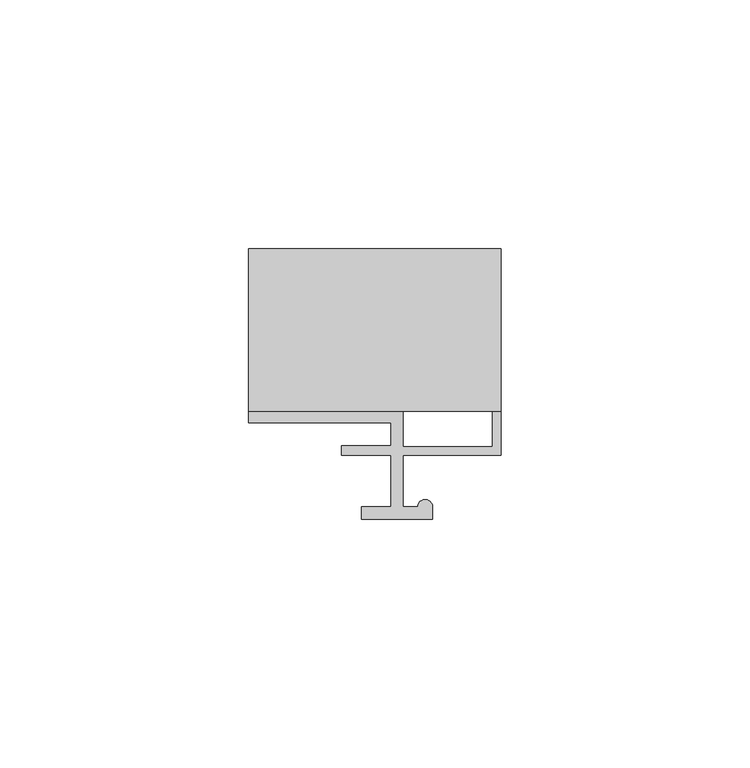
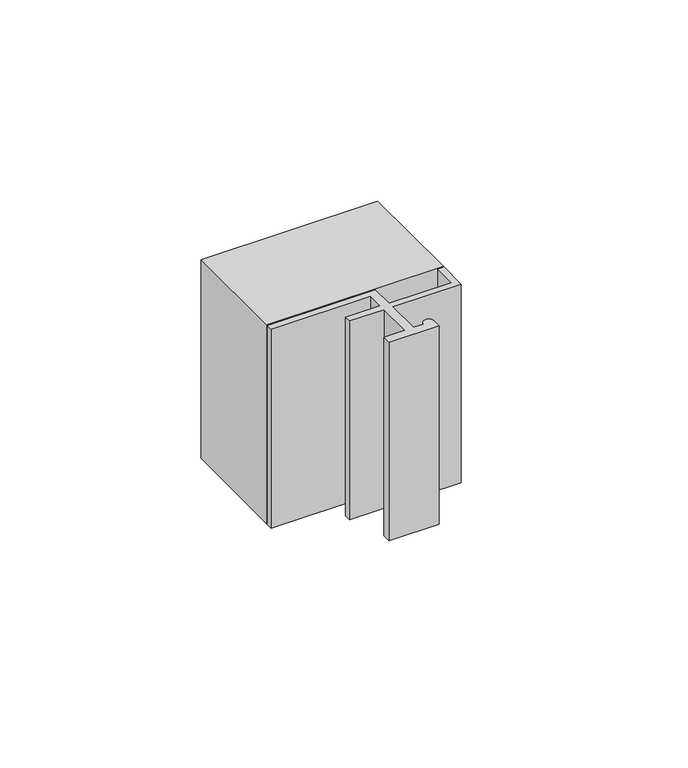
"""IFC4 building model written with IfcOpenShell, lengths in millimetres: proxy geometry, Generic Models 9:Generic Models 5:348123:Generic Models 5:348123 : Generic Models 9:Generic Models 5:348123:2 : Generic Models 9:Generic Models 5:348123:Generic Models 5:348123 : Generic Models 9:Generic Models 5:348123:301771."""

import ifcopenshell
import ifcopenshell.guid

model = None  # the IFC model being written
_history = None  # IfcOwnerHistory: only IFC2X3 demands one
_inside = {}  # id of a spatial element -> (the spatial element, [elements in it])
_under = {}  # id of a project, library or spatial element -> (it, [spatial elements below it])
_declared = {}  # id of a project -> (the project, [libraries it declares])
_typed = {}  # id of a type object -> (the type object, [elements of that type])
_made_of = {}  # id of a material, layer set ... -> (it, [elements and type objects made of it])


def new_model(schema):
    """Start an empty IFC model of exactly this schema.

    Asked for "IFC4X3", IfcOpenShell would pick the latest addendum, in which some entities
    have other attributes; the version numbers below select the first issue.
    IFC2X3 requires an IfcOwnerHistory on every rooted entity: one is made here for all.
    """
    global model, _history
    if schema == "IFC4X3":
        model = ifcopenshell.file(schema_version=(4, 3, 0, 0))
    else:
        model = ifcopenshell.file(schema=schema)
    _inside.clear()
    _under.clear()
    _declared.clear()
    _typed.clear()
    _made_of.clear()
    _history = None
    if model.schema == "IFC2X3":
        org = make("IfcOrganization", Name="unknown")
        user = make(
            "IfcPersonAndOrganization",
            ThePerson=make("IfcPerson", FamilyName="unknown"),
            TheOrganization=org,
        )
        app = make(
            "IfcApplication",
            ApplicationDeveloper=org,
            Version="unknown",
            ApplicationFullName="unknown",
            ApplicationIdentifier="unknown",
        )
        _history = make(
            "IfcOwnerHistory",
            OwningUser=user,
            OwningApplication=app,
            ChangeAction="ADDED",
            CreationDate=0,
        )
    return model


def make(cls, **values):
    """One entity of the class cls with the attributes given. An attribute that is None is left unset."""
    return model.create_entity(
        cls, **{name: value for name, value in values.items() if value is not None}
    )


def rooted(cls, **values):
    """An entity with a GlobalId (a new one), such as an element, a storey or a relation."""
    return make(cls, GlobalId=ifcopenshell.guid.new(), OwnerHistory=_history, **values)


def si_unit(unit_type, name, prefix=None):
    """IfcSIUnit, for example si_unit("LENGTHUNIT", "METRE", prefix="MILLI")."""
    return make("IfcSIUnit", UnitType=unit_type, Prefix=prefix, Name=name)


def assignment(units):
    """IfcUnitAssignment: the units of a project."""
    return None if units is None else make("IfcUnitAssignment", Units=units)


def point(xyz):
    """IfcCartesianPoint."""
    return None if xyz is None else make("IfcCartesianPoint", Coordinates=xyz)


def direction(xyz):
    """IfcDirection."""
    return None if xyz is None else make("IfcDirection", DirectionRatios=xyz)


def frame(location, z_axis=None, x_axis=None):
    """IfcAxis2Placement3D, a coordinate frame: its origin and axes. An axis left out is left unset."""
    return make(
        "IfcAxis2Placement3D",
        Location=point(location),
        Axis=direction(z_axis),
        RefDirection=direction(x_axis),
    )


def frame_2d(location, x_axis=None):
    """IfcAxis2Placement2D, a coordinate frame in the plane: its origin and x axis."""
    return make(
        "IfcAxis2Placement2D", Location=point(location), RefDirection=direction(x_axis)
    )


def origin():
    """The frame at (0, 0, 0) with its axes left unset."""
    return frame((0.0, 0.0, 0.0))


def place(relative_to, where):
    """IfcLocalPlacement: puts the frame where relative to a parent placement (None: the world)."""
    return make(
        "IfcLocalPlacement", PlacementRelTo=relative_to, RelativePlacement=where
    )


def context(
    kind, dimensions, precision=None, world=None, true_north=None, identifier=None
):
    """IfcGeometricRepresentationContext, for example the 3D "Model" context."""
    return make(
        "IfcGeometricRepresentationContext",
        ContextIdentifier=identifier,
        ContextType=kind,
        CoordinateSpaceDimension=dimensions,
        Precision=precision,
        WorldCoordinateSystem=world,
        TrueNorth=true_north,
    )


def project(units=None, contexts=None):
    """IfcProject with its units and contexts."""
    return rooted(
        "IfcProject",
        Name="project",
        RepresentationContexts=contexts,
        UnitsInContext=assignment(units),
    )


def spatial(cls, under=None, at=None, **own):
    """A site, building, storey or space (cls), placed at a placement, below another one or the project."""
    s = rooted(cls, ObjectPlacement=at, **own)
    if under is not None:
        _under.setdefault(under.id(), (under, []))[1].append(s)
    return s


def polyline(points):
    """IfcPolyline through the points."""
    return make("IfcPolyline", Points=[point(p) for p in points])


def circle_curve(where, radius):
    """IfcCircle in the frame where."""
    return make("IfcCircle", Position=where, Radius=radius)


def trimmed(basis, trim1, trim2, sense, master):
    """IfcTrimmedCurve: the piece of a basis curve between two trims."""
    return make(
        "IfcTrimmedCurve",
        BasisCurve=basis,
        Trim1=trim1,
        Trim2=trim2,
        SenseAgreement=sense,
        MasterRepresentation=master,
    )


def segment(curve, same_sense, transition):
    """IfcCompositeCurveSegment."""
    return make(
        "IfcCompositeCurveSegment",
        Transition=transition,
        SameSense=same_sense,
        ParentCurve=curve,
    )


def composite_curve(segments, self_intersect=None):
    """IfcCompositeCurve: segments joined end to end."""
    return make("IfcCompositeCurve", Segments=segments, SelfIntersect=self_intersect)


def outline(outer, holes=None, kind="AREA"):
    """IfcArbitraryClosedProfileDef: a profile drawn as a closed curve; with holes, ...WithVoids."""
    if holes is None:
        return make("IfcArbitraryClosedProfileDef", ProfileType=kind, OuterCurve=outer)
    return make(
        "IfcArbitraryProfileDefWithVoids",
        ProfileType=kind,
        OuterCurve=outer,
        InnerCurves=holes,
    )


def extrude(swept, where, along, depth):
    """IfcExtrudedAreaSolid: the profile swept, set in the frame where, extruded along a direction by depth."""
    return make(
        "IfcExtrudedAreaSolid",
        SweptArea=swept,
        Position=where,
        ExtrudedDirection=direction(along),
        Depth=depth,
    )


def shape(context_of_items, identifier, shape_type, items):
    """IfcShapeRepresentation: the items that make up one representation, for example the "Body"."""
    return make(
        "IfcShapeRepresentation",
        ContextOfItems=context_of_items,
        RepresentationIdentifier=identifier,
        RepresentationType=shape_type,
        Items=items,
    )


def source(mapping_origin, context_of_items, identifier, shape_type, items):
    """IfcRepresentationMap: a shape defined once, which mapped items show again and again."""
    return make(
        "IfcRepresentationMap",
        MappingOrigin=mapping_origin,
        MappedRepresentation=shape(context_of_items, identifier, shape_type, items),
    )


def transform(
    local_origin,
    x_axis=None,
    y_axis=None,
    z_axis=None,
    scale=None,
    scale2=None,
    scale3=None,
    uniform=True,
):
    """IfcCartesianTransformationOperator3D, or its non-uniform kind. x_axis, y_axis, z_axis: its Axis1, 2, 3."""
    if uniform:
        return make(
            "IfcCartesianTransformationOperator3D",
            Axis1=direction(x_axis),
            Axis2=direction(y_axis),
            LocalOrigin=point(local_origin),
            Scale=scale,
            Axis3=direction(z_axis),
        )
    return make(
        "IfcCartesianTransformationOperator3DnonUniform",
        Axis1=direction(x_axis),
        Axis2=direction(y_axis),
        LocalOrigin=point(local_origin),
        Scale=scale,
        Axis3=direction(z_axis),
        Scale2=scale2,
        Scale3=scale3,
    )


def mapped(mapping_source, mapping_target):
    """IfcMappedItem: shows the shape of a source again, moved by a transform."""
    return make(
        "IfcMappedItem", MappingSource=mapping_source, MappingTarget=mapping_target
    )


def made_of(thing, what):
    """Note that an element or type object is made of a material, layer set ...; save() writes the relation."""
    if what is not None:
        _made_of.setdefault(what.id(), (what, []))[1].append(thing)
    return thing


def element(
    cls,
    number,
    at=None,
    inside=None,
    cuts=None,
    type_object=None,
    material=None,
    context=None,
    identifier="Body",
    shape_type=None,
    held_by="IfcProductDefinitionShape",
    body=None,
    shapes=None,
    **own,
):
    """One element of the class cls, such as IfcWall. Its Tag is "e" and its number.

    at: its placement. inside: the storey or other place that contains it. cuts: it is an
    opening in that element (IfcRelVoidsElement). A single representation is given by context,
    identifier, shape_type and body (its items); several are given by shapes. held_by: the class
    of the entity that holds the representations. save() writes the other relations.
    """
    e = rooted(cls, Tag="e%d" % number, ObjectPlacement=at, **own)
    if body is not None:
        shapes = [shape(context, identifier, shape_type, body)]
    if shapes is not None:
        e.Representation = make(held_by, Representations=shapes)
    if inside is not None:
        _inside.setdefault(inside.id(), (inside, []))[1].append(e)
    if cuts is not None:
        rooted(
            "IfcRelVoidsElement", RelatingBuildingElement=cuts, RelatedOpeningElement=e
        )
    if type_object is not None:
        _typed.setdefault(type_object.id(), (type_object, []))[1].append(e)
    return made_of(e, material)


def aggregate(whole, parts):
    """IfcRelAggregates: a whole, such as a stair, and the parts it consists of."""
    return rooted("IfcRelAggregates", RelatingObject=whole, RelatedObjects=parts)


def save(model, path):
    """Write the relations noted so far, then the file.

    IfcRelAggregates (storeys below a building ...), IfcRelContainedInSpatialStructure (elements
    in a storey), IfcRelDefinesByType, IfcRelAssociatesMaterial and IfcRelDeclares: one each for
    every whole, place, type object, material and project.
    """
    for whole, parts in _under.values():
        aggregate(whole, parts)
    for where, things in _inside.values():
        rooted(
            "IfcRelContainedInSpatialStructure",
            RelatedElements=things,
            RelatingStructure=where,
        )
    for kind, things in _typed.values():
        rooted("IfcRelDefinesByType", RelatedObjects=things, RelatingType=kind)
    for what, things in _made_of.values():
        rooted("IfcRelAssociatesMaterial", RelatedObjects=things, RelatingMaterial=what)
    for by, libraries in _declared.values():
        rooted("IfcRelDeclares", RelatingContext=by, RelatedDefinitions=libraries)
    model.write(path)


def generic_models_f7c776a6(model_context):
    return source(origin(), model_context, "Body", "SweptSolid", [
        extrude(outline(polyline([(592204.7959377, -579000.6913841), (592255.5959377, -579000.6913841), (592255.5959377, -579033.3483921), (592204.7959377, -579033.3483921), (592204.7959377, -579000.6913841)])), frame((0.0, 0.0, 2458.6225209), z_axis=(0.0, 0.0, 1.0), x_axis=(1.0, 0.0, 0.0)), (0.0, 0.0, 1.0), 60.325),
        extrude(outline(composite_curve([segment(polyline([(592235.8677824, -579042.226062), (592235.8677824, -579052.5833435), (592238.8270057, -579052.5833435)]), True, "CONTINUOUS"), segment(trimmed(circle_curve(frame_2d((592240.3066173, -579052.5833435)), 1.4796117), [point((592238.8270057, -579052.5833435))], [point((592241.786229, -579052.5833435))], False, "CARTESIAN"), True, "CONTINUOUS"), segment(polyline([(592241.786229, -579052.5833435), (592241.786229, -579055.0493629), (592227.4833163, -579055.0493629), (592227.4833163, -579052.5833435), (592233.4017629, -579052.5833435), (592233.4017629, -579042.226062), (592223.5376853, -579042.226062), (592223.5376853, -579040.2532464), (592233.4017629, -579040.2532464), (592233.4017629, -579035.6171299), (592204.7959377, -579035.6171299), (592204.7959377, -579033.3483921), (592235.8677824, -579033.3483921), (592235.8677824, -579040.450528), (592253.8204037, -579040.450528), (592253.8204037, -579033.3483921), (592255.5959377, -579033.3483921), (592255.5959377, -579042.226062), (592235.8677824, -579042.226062)]), True, "CONTINUOUS")], self_intersect=False)), frame((0.0, 0.0, 2458.6225209), z_axis=(0.0, 0.0, 1.0), x_axis=(1.0, 0.0, 0.0)), (0.0, 0.0, 1.0), 60.325),
    ])


if __name__ == "__main__":
    model = new_model("IFC4")
    model_context = context("Model", 3, world=origin())
    ifc_project = project(units=[si_unit("LENGTHUNIT", "METRE", prefix="MILLI")], contexts=[model_context])
    site = spatial("IfcSite", under=ifc_project)
    building = spatial("IfcBuilding", under=site)
    placement = place(None, origin())
    generic_models_shape = generic_models_f7c776a6(model_context)
    element("IfcBuildingElementProxy", 1, Name="Generic Models 9:Generic Models 5:348123:Generic Models 5:348123 : Generic Models 9:Generic Models 5:348123:2 : Generic Models 9:Generic Models 5:348123:Generic Models 5:348123 : Generic Models 9:Generic Models 5:348123:301771", ObjectType="Generic Models 9:Generic Models 5:348123:Generic Models 5:348123 : Generic Models 9:Generic Models 5:348123:2 : Generic Models 9:Generic Models 5:348123:Generic Models 5:348123 : Generic Models 9:Generic Models 5:348123:301771", at=placement, inside=building, context=model_context, shape_type="MappedRepresentation", body=[
        mapped(generic_models_shape, transform((0.0, 0.0, 0.0), x_axis=(1.0, 0.0, 0.0), y_axis=(0.0, 1.0, 0.0), z_axis=(0.0, 0.0, 1.0))),
    ])
    save(model, "model.ifc")

# Revit data of these elements
# Type "Generic Models 9:Generic Models 5:348123:Generic Models 5:348123 : Generic Models 9:Generic Models 5:348123:2 : Generic Models 9:Generic Models 5:348123:Generic Models 5:348123 : Generic Models 9:Generic Models 5:348123:301771"
#   NameOverride = "Generic Models 9:Generic Models 5:348123:Generic Models 5:348123 : Generic Models 9:Generic Models 5:348123:301771"
#   ObjectTypeOverride = "Generic Models 5:348123 : Generic Models 9:Generic Models 5:348123"
#   Reference = "Generic Models 5"
#   Tag = "301771"
# Element 1 (IfcBuildingElementProxy, "Generic Models 9:Generic Models 5:348123:Generic Models 5:348123 : Generic Models 9:Generic Models 5:348123:2 : Generic Models 9:Generic Models 5:348123:Generic Models 5:348123 : Generic Models 9:Generic Models 5:348123:301771")
#   Materials on its faces: "GALVANIZED STEEL CLIP AT EVERY SEAM IN POLYCARBONATE"
# Materials
#   "GALVANIZED STEEL CLIP AT EVERY SEAM IN POLYCARBONATE": class "Unassigned", colour RGB 120 120 120, transparency 0, Cost = 0
